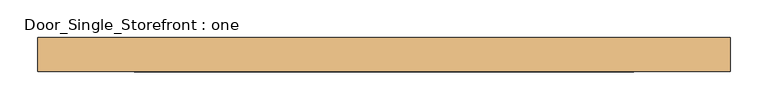
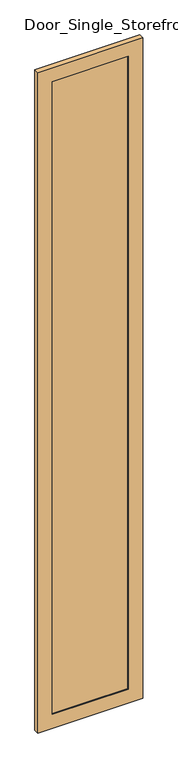
"""IFC4 building model written with IfcOpenShell, lengths in millimetres: door geometry, Door_Single_Storefront : one."""

from ifc_helpers import new_model, si_unit, frame, origin, place, context, project, spatial, polyline, outline, extrude, source, transform, mapped, element, save


def door_single_storefront_one_4252a597(model_context):
    return source(origin(), model_context, "Body", "SweptSolid", [
        extrude(outline(polyline([(330.2, 6.35), (330.2, -12.7), (-330.2, -12.7), (-330.2, 6.35), (330.2, 6.35)])), frame((0.0, 0.0, 127.0), z_axis=(0.0, 0.0, 1.0), x_axis=(1.0, 0.0, 0.0)), (0.0, 0.0, 1.0), 5835.65),
        extrude(outline(polyline([(6089.65, -457.2), (0.0, -457.2), (0.0, 457.2), (6089.65, 457.2), (6089.65, -457.2)]), holes=[polyline([(127.0, 330.2), (127.0, -330.2), (5962.65, -330.2), (5962.65, 330.2), (127.0, 330.2)])]), frame((0.0, -25.4, 0.0), z_axis=(0.0, 1.0, 0.0), x_axis=(0.0, 0.0, 1.0)), (0.0, 0.0, 1.0), 44.45),
    ])


if __name__ == "__main__":
    model = new_model("IFC4")
    model_context = context("Model", 3, world=origin())
    ifc_project = project(units=[si_unit("LENGTHUNIT", "METRE", prefix="MILLI")], contexts=[model_context])
    site = spatial("IfcSite", under=ifc_project)
    building = spatial("IfcBuilding", under=site)
    placement = place(None, origin())
    door_single_storefront_one_shape = door_single_storefront_one_4252a597(model_context)
    element("IfcDoor", 1, ObjectType="Door_Single_Storefront : one", at=placement, inside=building, context=model_context, shape_type="MappedRepresentation", body=[
        mapped(door_single_storefront_one_shape, transform((0.0, 0.0, 0.0), x_axis=(1.0, 0.0, 0.0), y_axis=(0.0, 1.0, 0.0), z_axis=(0.0, 0.0, 1.0))),
    ])
    save(model, "model.ifc")

# Revit data of these elements
# Type "Door_Single_Storefront : one"
#   Type Mark = "107"
#   Analytic Construction = "<None>"
#   Stile_Width = 0' - 5"
#   Door_Thickness = 0' - 1 3/4"
#   Door_Offset = 0' - 1"
#   Glass_Material = TEMPERED, INSULATED GLASS
#   Frame_Material = EXISTING STOREFRONT
#   Function = (empty or 0)
# Element 1 (IfcDoor, "Door_Single_Storefront : one")
#   Materials on its faces: "EXISTING STOREFRONT", "TEMPERED, INSULATED GLASS"
# Materials
#   "TEMPERED, INSULATED GLASS": class "Glass", colour RGB 214 219 226, transparency 0, Description = "Soda Lime Glass", Cost = 0
#   "EXISTING STOREFRONT": class "Metal", colour RGB 244 244 244, transparency 0, Description = "Aluminum 6061", Cost = 0
